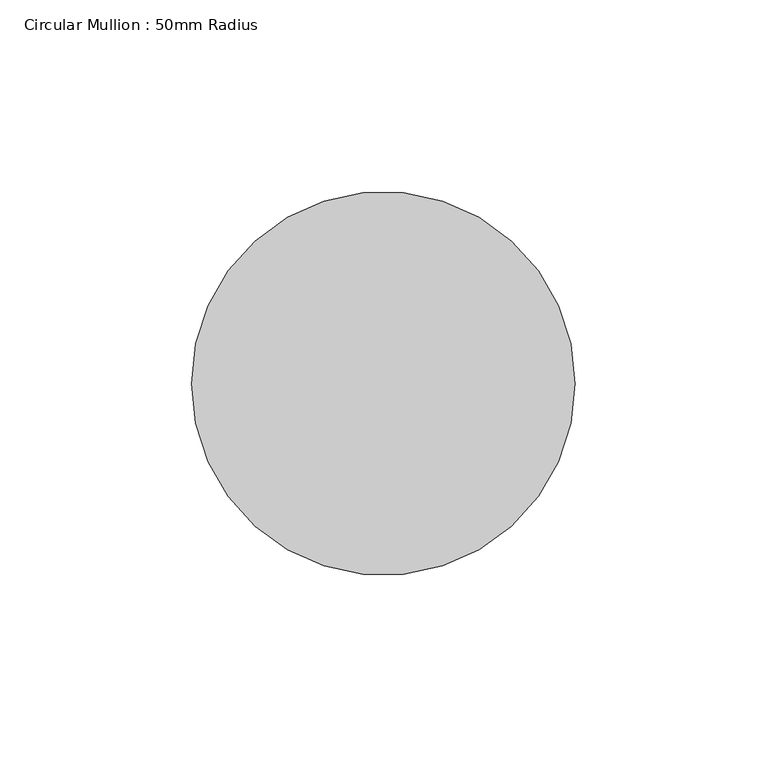
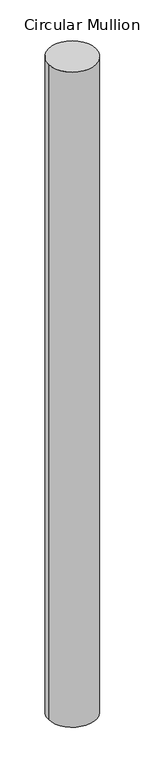
"""IFC4 building model written with IfcOpenShell, lengths in millimetres: member geometry, Circular Mullion : 50mm Radius."""

from ifc_helpers import new_model, si_unit, point, frame, origin, origin_2d, place, context, project, spatial, circle_curve, trimmed, segment, composite_curve, outline, extrude, source, transform, mapped, element, save


def circular_mullion_50mm_radius_ab774a8e(model_context):
    return source(origin(), model_context, "Body", "SweptSolid", [
        extrude(outline(composite_curve([segment(trimmed(circle_curve(origin_2d(), 50.0), [point((50.0, 0.0))], [point((-50.0, 0.0))], False, "CARTESIAN"), True, "CONTINUOUS"), segment(trimmed(circle_curve(origin_2d(), 50.0), [point((-50.0, 0.0))], [point((50.0, 0.0))], False, "CARTESIAN"), True, "CONTINUOUS")], self_intersect=False)), frame((0.0, 0.0, -1452.5117446), z_axis=(0.0, 0.0, 1.0), x_axis=(1.0, 0.0, 0.0)), (0.0, 0.0, 1.0), 1452.5117446),
    ])


if __name__ == "__main__":
    model = new_model("IFC4")
    model_context = context("Model", 3, world=origin())
    ifc_project = project(units=[si_unit("LENGTHUNIT", "METRE", prefix="MILLI")], contexts=[model_context])
    site = spatial("IfcSite", under=ifc_project)
    building = spatial("IfcBuilding", under=site)
    placement = place(None, origin())
    circular_mullion_50mm_radius_shape = circular_mullion_50mm_radius_ab774a8e(model_context)
    element("IfcMember", 1, ObjectType="Circular Mullion : 50mm Radius", at=placement, inside=building, context=model_context, shape_type="MappedRepresentation", body=[
        mapped(circular_mullion_50mm_radius_shape, transform((0.0, 0.0, 0.0), x_axis=(1.0, 0.0, 0.0), y_axis=(0.0, 1.0, 0.0), z_axis=(0.0, 0.0, 1.0))),
    ])
    save(model, "model.ifc")

# Revit data of these elements
# Type "Circular Mullion : 50mm Radius"
#   built-in parameter 1007350 = 0.164042 (stored number, unit not read)
# Element 1 (IfcMember, "Circular Mullion : 50mm Radius")
#   Materials on its faces: "Aluminium"
# Materials
#   "Aluminium": class "Metal", colour RGB 247 247 247, transparency 0, Description = "Aluminium 6061", Cost = 0
